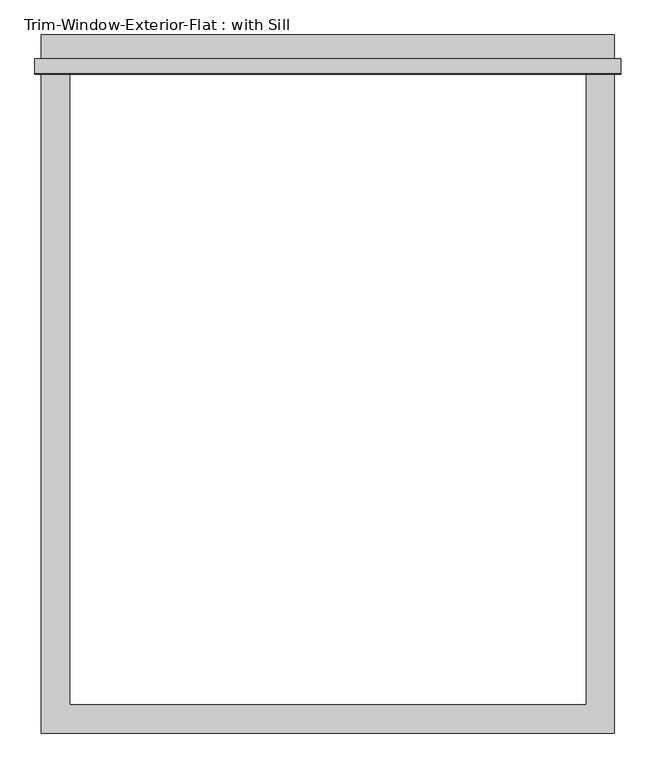
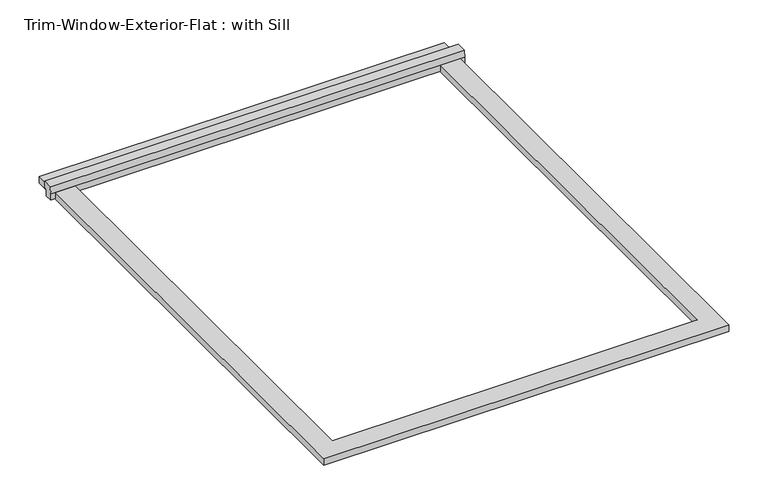
"""IFC4 building model written with IfcOpenShell, lengths in millimetres: proxy geometry, Trim-Window-Exterior-Flat : with Sill."""

import ifcopenshell
import ifcopenshell.guid

model = None  # the IFC model being written
_history = None  # IfcOwnerHistory: only IFC2X3 demands one
_inside = {}  # id of a spatial element -> (the spatial element, [elements in it])
_under = {}  # id of a project, library or spatial element -> (it, [spatial elements below it])
_declared = {}  # id of a project -> (the project, [libraries it declares])
_typed = {}  # id of a type object -> (the type object, [elements of that type])
_made_of = {}  # id of a material, layer set ... -> (it, [elements and type objects made of it])


def new_model(schema):
    """Start an empty IFC model of exactly this schema.

    Asked for "IFC4X3", IfcOpenShell would pick the latest addendum, in which some entities
    have other attributes; the version numbers below select the first issue.
    IFC2X3 requires an IfcOwnerHistory on every rooted entity: one is made here for all.
    """
    global model, _history
    if schema == "IFC4X3":
        model = ifcopenshell.file(schema_version=(4, 3, 0, 0))
    else:
        model = ifcopenshell.file(schema=schema)
    _inside.clear()
    _under.clear()
    _declared.clear()
    _typed.clear()
    _made_of.clear()
    _history = None
    if model.schema == "IFC2X3":
        org = make("IfcOrganization", Name="unknown")
        user = make(
            "IfcPersonAndOrganization",
            ThePerson=make("IfcPerson", FamilyName="unknown"),
            TheOrganization=org,
        )
        app = make(
            "IfcApplication",
            ApplicationDeveloper=org,
            Version="unknown",
            ApplicationFullName="unknown",
            ApplicationIdentifier="unknown",
        )
        _history = make(
            "IfcOwnerHistory",
            OwningUser=user,
            OwningApplication=app,
            ChangeAction="ADDED",
            CreationDate=0,
        )
    return model


def make(cls, **values):
    """One entity of the class cls with the attributes given. An attribute that is None is left unset."""
    return model.create_entity(
        cls, **{name: value for name, value in values.items() if value is not None}
    )


def rooted(cls, **values):
    """An entity with a GlobalId (a new one), such as an element, a storey or a relation."""
    return make(cls, GlobalId=ifcopenshell.guid.new(), OwnerHistory=_history, **values)


def si_unit(unit_type, name, prefix=None):
    """IfcSIUnit, for example si_unit("LENGTHUNIT", "METRE", prefix="MILLI")."""
    return make("IfcSIUnit", UnitType=unit_type, Prefix=prefix, Name=name)


def assignment(units):
    """IfcUnitAssignment: the units of a project."""
    return None if units is None else make("IfcUnitAssignment", Units=units)


def point(xyz):
    """IfcCartesianPoint."""
    return None if xyz is None else make("IfcCartesianPoint", Coordinates=xyz)


def direction(xyz):
    """IfcDirection."""
    return None if xyz is None else make("IfcDirection", DirectionRatios=xyz)


def frame(location, z_axis=None, x_axis=None):
    """IfcAxis2Placement3D, a coordinate frame: its origin and axes. An axis left out is left unset."""
    return make(
        "IfcAxis2Placement3D",
        Location=point(location),
        Axis=direction(z_axis),
        RefDirection=direction(x_axis),
    )


def origin():
    """The frame at (0, 0, 0) with its axes left unset."""
    return frame((0.0, 0.0, 0.0))


def origin_with_axes():
    """The frame at (0, 0, 0) with the z axis (0, 0, 1) and the x axis (1, 0, 0) written out."""
    return frame((0.0, 0.0, 0.0), z_axis=(0.0, 0.0, 1.0), x_axis=(1.0, 0.0, 0.0))


def place(relative_to, where):
    """IfcLocalPlacement: puts the frame where relative to a parent placement (None: the world)."""
    return make(
        "IfcLocalPlacement", PlacementRelTo=relative_to, RelativePlacement=where
    )


def context(
    kind, dimensions, precision=None, world=None, true_north=None, identifier=None
):
    """IfcGeometricRepresentationContext, for example the 3D "Model" context."""
    return make(
        "IfcGeometricRepresentationContext",
        ContextIdentifier=identifier,
        ContextType=kind,
        CoordinateSpaceDimension=dimensions,
        Precision=precision,
        WorldCoordinateSystem=world,
        TrueNorth=true_north,
    )


def project(units=None, contexts=None):
    """IfcProject with its units and contexts."""
    return rooted(
        "IfcProject",
        Name="project",
        RepresentationContexts=contexts,
        UnitsInContext=assignment(units),
    )


def spatial(cls, under=None, at=None, **own):
    """A site, building, storey or space (cls), placed at a placement, below another one or the project."""
    s = rooted(cls, ObjectPlacement=at, **own)
    if under is not None:
        _under.setdefault(under.id(), (under, []))[1].append(s)
    return s


def polyline(points):
    """IfcPolyline through the points."""
    return make("IfcPolyline", Points=[point(p) for p in points])


def outline(outer, holes=None, kind="AREA"):
    """IfcArbitraryClosedProfileDef: a profile drawn as a closed curve; with holes, ...WithVoids."""
    if holes is None:
        return make("IfcArbitraryClosedProfileDef", ProfileType=kind, OuterCurve=outer)
    return make(
        "IfcArbitraryProfileDefWithVoids",
        ProfileType=kind,
        OuterCurve=outer,
        InnerCurves=holes,
    )


def extrude(swept, where, along, depth):
    """IfcExtrudedAreaSolid: the profile swept, set in the frame where, extruded along a direction by depth."""
    return make(
        "IfcExtrudedAreaSolid",
        SweptArea=swept,
        Position=where,
        ExtrudedDirection=direction(along),
        Depth=depth,
    )


def shape(context_of_items, identifier, shape_type, items):
    """IfcShapeRepresentation: the items that make up one representation, for example the "Body"."""
    return make(
        "IfcShapeRepresentation",
        ContextOfItems=context_of_items,
        RepresentationIdentifier=identifier,
        RepresentationType=shape_type,
        Items=items,
    )


def source(mapping_origin, context_of_items, identifier, shape_type, items):
    """IfcRepresentationMap: a shape defined once, which mapped items show again and again."""
    return make(
        "IfcRepresentationMap",
        MappingOrigin=mapping_origin,
        MappedRepresentation=shape(context_of_items, identifier, shape_type, items),
    )


def transform(
    local_origin,
    x_axis=None,
    y_axis=None,
    z_axis=None,
    scale=None,
    scale2=None,
    scale3=None,
    uniform=True,
):
    """IfcCartesianTransformationOperator3D, or its non-uniform kind. x_axis, y_axis, z_axis: its Axis1, 2, 3."""
    if uniform:
        return make(
            "IfcCartesianTransformationOperator3D",
            Axis1=direction(x_axis),
            Axis2=direction(y_axis),
            LocalOrigin=point(local_origin),
            Scale=scale,
            Axis3=direction(z_axis),
        )
    return make(
        "IfcCartesianTransformationOperator3DnonUniform",
        Axis1=direction(x_axis),
        Axis2=direction(y_axis),
        LocalOrigin=point(local_origin),
        Scale=scale,
        Axis3=direction(z_axis),
        Scale2=scale2,
        Scale3=scale3,
    )


def mapped(mapping_source, mapping_target):
    """IfcMappedItem: shows the shape of a source again, moved by a transform."""
    return make(
        "IfcMappedItem", MappingSource=mapping_source, MappingTarget=mapping_target
    )


def made_of(thing, what):
    """Note that an element or type object is made of a material, layer set ...; save() writes the relation."""
    if what is not None:
        _made_of.setdefault(what.id(), (what, []))[1].append(thing)
    return thing


def element(
    cls,
    number,
    at=None,
    inside=None,
    cuts=None,
    type_object=None,
    material=None,
    context=None,
    identifier="Body",
    shape_type=None,
    held_by="IfcProductDefinitionShape",
    body=None,
    shapes=None,
    **own,
):
    """One element of the class cls, such as IfcWall. Its Tag is "e" and its number.

    at: its placement. inside: the storey or other place that contains it. cuts: it is an
    opening in that element (IfcRelVoidsElement). A single representation is given by context,
    identifier, shape_type and body (its items); several are given by shapes. held_by: the class
    of the entity that holds the representations. save() writes the other relations.
    """
    e = rooted(cls, Tag="e%d" % number, ObjectPlacement=at, **own)
    if body is not None:
        shapes = [shape(context, identifier, shape_type, body)]
    if shapes is not None:
        e.Representation = make(held_by, Representations=shapes)
    if inside is not None:
        _inside.setdefault(inside.id(), (inside, []))[1].append(e)
    if cuts is not None:
        rooted(
            "IfcRelVoidsElement", RelatingBuildingElement=cuts, RelatedOpeningElement=e
        )
    if type_object is not None:
        _typed.setdefault(type_object.id(), (type_object, []))[1].append(e)
    return made_of(e, material)


def aggregate(whole, parts):
    """IfcRelAggregates: a whole, such as a stair, and the parts it consists of."""
    return rooted("IfcRelAggregates", RelatingObject=whole, RelatedObjects=parts)


def save(model, path):
    """Write the relations noted so far, then the file.

    IfcRelAggregates (storeys below a building ...), IfcRelContainedInSpatialStructure (elements
    in a storey), IfcRelDefinesByType, IfcRelAssociatesMaterial and IfcRelDeclares: one each for
    every whole, place, type object, material and project.
    """
    for whole, parts in _under.values():
        aggregate(whole, parts)
    for where, things in _inside.values():
        rooted(
            "IfcRelContainedInSpatialStructure",
            RelatedElements=things,
            RelatingStructure=where,
        )
    for kind, things in _typed.values():
        rooted("IfcRelDefinesByType", RelatedObjects=things, RelatingType=kind)
    for what, things in _made_of.values():
        rooted("IfcRelAssociatesMaterial", RelatedObjects=things, RelatingMaterial=what)
    for by, libraries in _declared.values():
        rooted("IfcRelDeclares", RelatingContext=by, RelatedDefinitions=libraries)
    model.write(path)


def trim_window_exterior_flat_with_sill_256f2652(model_context):
    return source(origin(), model_context, "Body", "SweptSolid", [
        extrude(outline(polyline([(577.85, 1292.1823709), (-577.85, 1292.1823709), (-577.85, 1349.3323709), (577.85, 1349.3323709), (577.85, 1292.1823709)])), origin_with_axes(), (0.0, 0.0, 1.0), 19.05),
        extrude(outline(polyline([(1301.75, 38.1), (1301.75, 19.05), (1292.1823709, 19.05), (1292.1823709, 0.0), (1270.0, 0.0), (1270.0, 19.05), (1272.4580645, 38.1), (1301.75, 38.1)])), frame((-590.55, 0.0, 0.0), z_axis=(1.0, 0.0, 0.0), x_axis=(0.0, 1.0, 0.0)), (0.0, 0.0, 1.0), 1181.1),
        extrude(outline(polyline([(-577.85, -57.15), (-577.85, 1270.0), (-520.7, 1270.0), (-520.7, 0.0), (520.7, 0.0), (520.7, 1270.0), (577.85, 1270.0), (577.85, -57.15), (-577.85, -57.15)])), origin_with_axes(), (0.0, 0.0, 1.0), 19.05),
    ])


if __name__ == "__main__":
    model = new_model("IFC4")
    model_context = context("Model", 3, world=origin())
    ifc_project = project(units=[si_unit("LENGTHUNIT", "METRE", prefix="MILLI")], contexts=[model_context])
    site = spatial("IfcSite", under=ifc_project)
    building = spatial("IfcBuilding", under=site)
    placement = place(None, origin())
    trim_window_exterior_flat_with_sill_shape = trim_window_exterior_flat_with_sill_256f2652(model_context)
    element("IfcBuildingElementProxy", 1, Name="Trim-Window-Exterior-Flat : with Sill", ObjectType="Trim-Window-Exterior-Flat : with Sill", at=placement, inside=building, context=model_context, shape_type="MappedRepresentation", body=[
        mapped(trim_window_exterior_flat_with_sill_shape, transform((0.0, 0.0, 0.0), x_axis=(1.0, 0.0, 0.0), y_axis=(0.0, 1.0, 0.0), z_axis=(0.0, 0.0, 1.0))),
    ])
    save(model, "model.ifc")

# Revit data of these elements
# Type "Trim-Window-Exterior-Flat : with Sill"
#   Trim Width = 0' - 2 1/4"
#   Trim Thickness_Picture Frame = 0' - 1 1/4"
#   Trim Thickness_with Sill = 0' - 0 3/4"
#   Sill Thickness = 0' - 1 1/4"
#   Opening Width [instance default] = 2' - 0"
#   Opening Height [instance default] = 3' - 0"
#   Default Elevation = 4' - 0"
#   Sill = yes
#   Picture Frame = no
#   Trim Material [instance default] = none
# Element 1 (IfcBuildingElementProxy, "Trim-Window-Exterior-Flat : with Sill")
#   Opening Width = 3' - 5"
#   Opening Height = 4' - 2"
#   Trim Material = Clad - White
#   Materials on its faces: "Clad - White"
# Materials
#   "Clad - White": class "Wood", colour RGB 242 242 238, transparency 0, Cost = 0
